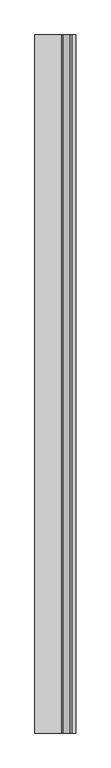
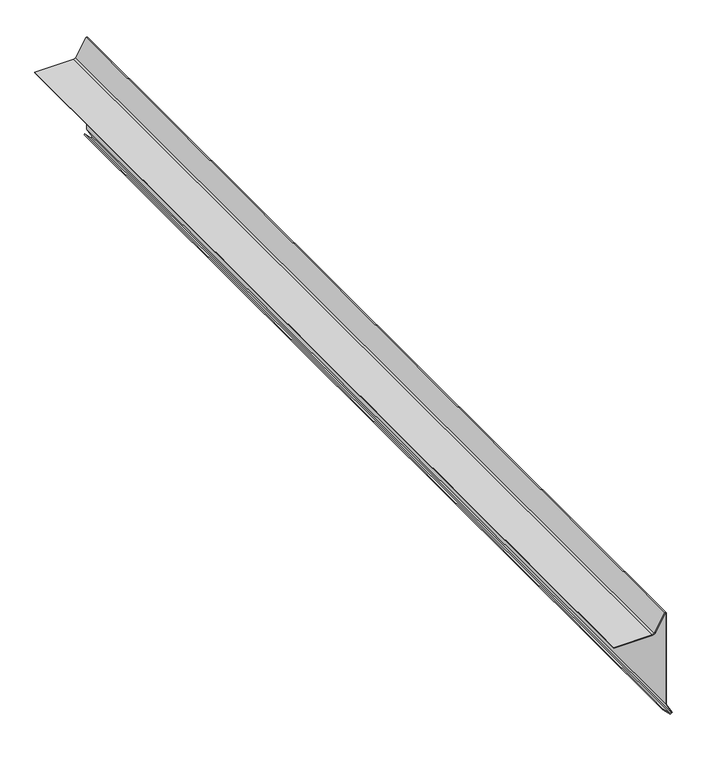
"""IFC4 building model written with IfcOpenShell, lengths in millimetres: proxy geometry, GRAVEL STOP005 3784 : GRAVEL STOP005 3784."""

import ifcopenshell
import ifcopenshell.guid

model = None  # the IFC model being written
_history = None  # IfcOwnerHistory: only IFC2X3 demands one
_inside = {}  # id of a spatial element -> (the spatial element, [elements in it])
_under = {}  # id of a project, library or spatial element -> (it, [spatial elements below it])
_declared = {}  # id of a project -> (the project, [libraries it declares])
_typed = {}  # id of a type object -> (the type object, [elements of that type])
_made_of = {}  # id of a material, layer set ... -> (it, [elements and type objects made of it])


def new_model(schema):
    """Start an empty IFC model of exactly this schema.

    Asked for "IFC4X3", IfcOpenShell would pick the latest addendum, in which some entities
    have other attributes; the version numbers below select the first issue.
    IFC2X3 requires an IfcOwnerHistory on every rooted entity: one is made here for all.
    """
    global model, _history
    if schema == "IFC4X3":
        model = ifcopenshell.file(schema_version=(4, 3, 0, 0))
    else:
        model = ifcopenshell.file(schema=schema)
    _inside.clear()
    _under.clear()
    _declared.clear()
    _typed.clear()
    _made_of.clear()
    _history = None
    if model.schema == "IFC2X3":
        org = make("IfcOrganization", Name="unknown")
        user = make(
            "IfcPersonAndOrganization",
            ThePerson=make("IfcPerson", FamilyName="unknown"),
            TheOrganization=org,
        )
        app = make(
            "IfcApplication",
            ApplicationDeveloper=org,
            Version="unknown",
            ApplicationFullName="unknown",
            ApplicationIdentifier="unknown",
        )
        _history = make(
            "IfcOwnerHistory",
            OwningUser=user,
            OwningApplication=app,
            ChangeAction="ADDED",
            CreationDate=0,
        )
    return model


def make(cls, **values):
    """One entity of the class cls with the attributes given. An attribute that is None is left unset."""
    return model.create_entity(
        cls, **{name: value for name, value in values.items() if value is not None}
    )


def rooted(cls, **values):
    """An entity with a GlobalId (a new one), such as an element, a storey or a relation."""
    return make(cls, GlobalId=ifcopenshell.guid.new(), OwnerHistory=_history, **values)


def si_unit(unit_type, name, prefix=None):
    """IfcSIUnit, for example si_unit("LENGTHUNIT", "METRE", prefix="MILLI")."""
    return make("IfcSIUnit", UnitType=unit_type, Prefix=prefix, Name=name)


def assignment(units):
    """IfcUnitAssignment: the units of a project."""
    return None if units is None else make("IfcUnitAssignment", Units=units)


def point(xyz):
    """IfcCartesianPoint."""
    return None if xyz is None else make("IfcCartesianPoint", Coordinates=xyz)


def direction(xyz):
    """IfcDirection."""
    return None if xyz is None else make("IfcDirection", DirectionRatios=xyz)


def frame(location, z_axis=None, x_axis=None):
    """IfcAxis2Placement3D, a coordinate frame: its origin and axes. An axis left out is left unset."""
    return make(
        "IfcAxis2Placement3D",
        Location=point(location),
        Axis=direction(z_axis),
        RefDirection=direction(x_axis),
    )


def origin():
    """The frame at (0, 0, 0) with its axes left unset."""
    return frame((0.0, 0.0, 0.0))


def place(relative_to, where):
    """IfcLocalPlacement: puts the frame where relative to a parent placement (None: the world)."""
    return make(
        "IfcLocalPlacement", PlacementRelTo=relative_to, RelativePlacement=where
    )


def context(
    kind, dimensions, precision=None, world=None, true_north=None, identifier=None
):
    """IfcGeometricRepresentationContext, for example the 3D "Model" context."""
    return make(
        "IfcGeometricRepresentationContext",
        ContextIdentifier=identifier,
        ContextType=kind,
        CoordinateSpaceDimension=dimensions,
        Precision=precision,
        WorldCoordinateSystem=world,
        TrueNorth=true_north,
    )


def project(units=None, contexts=None):
    """IfcProject with its units and contexts."""
    return rooted(
        "IfcProject",
        Name="project",
        RepresentationContexts=contexts,
        UnitsInContext=assignment(units),
    )


def spatial(cls, under=None, at=None, **own):
    """A site, building, storey or space (cls), placed at a placement, below another one or the project."""
    s = rooted(cls, ObjectPlacement=at, **own)
    if under is not None:
        _under.setdefault(under.id(), (under, []))[1].append(s)
    return s


def polyline(points):
    """IfcPolyline through the points."""
    return make("IfcPolyline", Points=[point(p) for p in points])


def outline(outer, holes=None, kind="AREA"):
    """IfcArbitraryClosedProfileDef: a profile drawn as a closed curve; with holes, ...WithVoids."""
    if holes is None:
        return make("IfcArbitraryClosedProfileDef", ProfileType=kind, OuterCurve=outer)
    return make(
        "IfcArbitraryProfileDefWithVoids",
        ProfileType=kind,
        OuterCurve=outer,
        InnerCurves=holes,
    )


def extrude(swept, where, along, depth):
    """IfcExtrudedAreaSolid: the profile swept, set in the frame where, extruded along a direction by depth."""
    return make(
        "IfcExtrudedAreaSolid",
        SweptArea=swept,
        Position=where,
        ExtrudedDirection=direction(along),
        Depth=depth,
    )


def shape(context_of_items, identifier, shape_type, items):
    """IfcShapeRepresentation: the items that make up one representation, for example the "Body"."""
    return make(
        "IfcShapeRepresentation",
        ContextOfItems=context_of_items,
        RepresentationIdentifier=identifier,
        RepresentationType=shape_type,
        Items=items,
    )


def source(mapping_origin, context_of_items, identifier, shape_type, items):
    """IfcRepresentationMap: a shape defined once, which mapped items show again and again."""
    return make(
        "IfcRepresentationMap",
        MappingOrigin=mapping_origin,
        MappedRepresentation=shape(context_of_items, identifier, shape_type, items),
    )


def transform(
    local_origin,
    x_axis=None,
    y_axis=None,
    z_axis=None,
    scale=None,
    scale2=None,
    scale3=None,
    uniform=True,
):
    """IfcCartesianTransformationOperator3D, or its non-uniform kind. x_axis, y_axis, z_axis: its Axis1, 2, 3."""
    if uniform:
        return make(
            "IfcCartesianTransformationOperator3D",
            Axis1=direction(x_axis),
            Axis2=direction(y_axis),
            LocalOrigin=point(local_origin),
            Scale=scale,
            Axis3=direction(z_axis),
        )
    return make(
        "IfcCartesianTransformationOperator3DnonUniform",
        Axis1=direction(x_axis),
        Axis2=direction(y_axis),
        LocalOrigin=point(local_origin),
        Scale=scale,
        Axis3=direction(z_axis),
        Scale2=scale2,
        Scale3=scale3,
    )


def mapped(mapping_source, mapping_target):
    """IfcMappedItem: shows the shape of a source again, moved by a transform."""
    return make(
        "IfcMappedItem", MappingSource=mapping_source, MappingTarget=mapping_target
    )


def made_of(thing, what):
    """Note that an element or type object is made of a material, layer set ...; save() writes the relation."""
    if what is not None:
        _made_of.setdefault(what.id(), (what, []))[1].append(thing)
    return thing


def element(
    cls,
    number,
    at=None,
    inside=None,
    cuts=None,
    type_object=None,
    material=None,
    context=None,
    identifier="Body",
    shape_type=None,
    held_by="IfcProductDefinitionShape",
    body=None,
    shapes=None,
    **own,
):
    """One element of the class cls, such as IfcWall. Its Tag is "e" and its number.

    at: its placement. inside: the storey or other place that contains it. cuts: it is an
    opening in that element (IfcRelVoidsElement). A single representation is given by context,
    identifier, shape_type and body (its items); several are given by shapes. held_by: the class
    of the entity that holds the representations. save() writes the other relations.
    """
    e = rooted(cls, Tag="e%d" % number, ObjectPlacement=at, **own)
    if body is not None:
        shapes = [shape(context, identifier, shape_type, body)]
    if shapes is not None:
        e.Representation = make(held_by, Representations=shapes)
    if inside is not None:
        _inside.setdefault(inside.id(), (inside, []))[1].append(e)
    if cuts is not None:
        rooted(
            "IfcRelVoidsElement", RelatingBuildingElement=cuts, RelatedOpeningElement=e
        )
    if type_object is not None:
        _typed.setdefault(type_object.id(), (type_object, []))[1].append(e)
    return made_of(e, material)


def aggregate(whole, parts):
    """IfcRelAggregates: a whole, such as a stair, and the parts it consists of."""
    return rooted("IfcRelAggregates", RelatingObject=whole, RelatedObjects=parts)


def save(model, path):
    """Write the relations noted so far, then the file.

    IfcRelAggregates (storeys below a building ...), IfcRelContainedInSpatialStructure (elements
    in a storey), IfcRelDefinesByType, IfcRelAssociatesMaterial and IfcRelDeclares: one each for
    every whole, place, type object, material and project.
    """
    for whole, parts in _under.values():
        aggregate(whole, parts)
    for where, things in _inside.values():
        rooted(
            "IfcRelContainedInSpatialStructure",
            RelatedElements=things,
            RelatingStructure=where,
        )
    for kind, things in _typed.values():
        rooted("IfcRelDefinesByType", RelatedObjects=things, RelatingType=kind)
    for what, things in _made_of.values():
        rooted("IfcRelAssociatesMaterial", RelatedObjects=things, RelatingMaterial=what)
    for by, libraries in _declared.values():
        rooted("IfcRelDeclares", RelatingContext=by, RelatedDefinitions=libraries)
    model.write(path)


def generic_models_bb7cdfd3(model_context):
    return source(origin(), model_context, "Body", "SweptSolid", [
        extrude(outline(polyline([(40077.410403, -4353.4420496), (40080.5182783, -4349.3681054), (40101.8558531, -4361.0170744), (40294.5307525, -4361.0170744), (40295.3431515, -4364.0489887), (40259.5408757, -4384.7194423), (40257.3744784, -4388.4717525), (40257.3744784, -4465.9296592), (40255.9633674, -4465.9296592), (40255.9633674, -4388.0936464), (40258.5078708, -4383.6864373), (40293.699878, -4363.3683225), (40293.447969, -4362.4281854), (40101.495749, -4362.4281854), (40080.9054201, -4351.1871656), (40079.2807815, -4353.3168157), (40092.8027062, -4366.8387404), (40091.8049, -4367.8365465), (40077.410403, -4353.4420496)])), frame((0.0, -1065.5906573, 0.0), z_axis=(0.0, 1.0, 0.0), x_axis=(0.0, 0.0, 1.0)), (0.0, 0.0, 1.0), 2000.25),
    ])


if __name__ == "__main__":
    model = new_model("IFC4")
    model_context = context("Model", 3, world=origin())
    ifc_project = project(units=[si_unit("LENGTHUNIT", "METRE", prefix="MILLI")], contexts=[model_context])
    site = spatial("IfcSite", under=ifc_project)
    building = spatial("IfcBuilding", under=site)
    placement = place(None, origin())
    generic_models_shape = generic_models_bb7cdfd3(model_context)
    element("IfcBuildingElementProxy", 1, Name="GRAVEL STOP005 3784 : GRAVEL STOP005 3784", ObjectType="GRAVEL STOP005 3784 : GRAVEL STOP005 3784", at=placement, inside=building, context=model_context, shape_type="MappedRepresentation", body=[
        mapped(generic_models_shape, transform((0.0, 0.0, 0.0), x_axis=(1.0, 0.0, 0.0), y_axis=(0.0, 1.0, 0.0), z_axis=(0.0, 0.0, 1.0))),
    ])
    save(model, "model.ifc")

# Revit data of these elements
# Type "GRAVEL STOP005 3784 : GRAVEL STOP005 3784"
#   NameOverride = "GRAVEL STOP005"
# Element 1 (IfcBuildingElementProxy, "GRAVEL STOP005 3784 : GRAVEL STOP005 3784")
#   Materials on its faces: "GRAVEL STOP REQUIRED WITH GRAVEL SURFACE SYSTEMS"
# Materials
#   "GRAVEL STOP REQUIRED WITH GRAVEL SURFACE SYSTEMS": class "Unassigned", colour RGB 170 170 127, transparency 0
